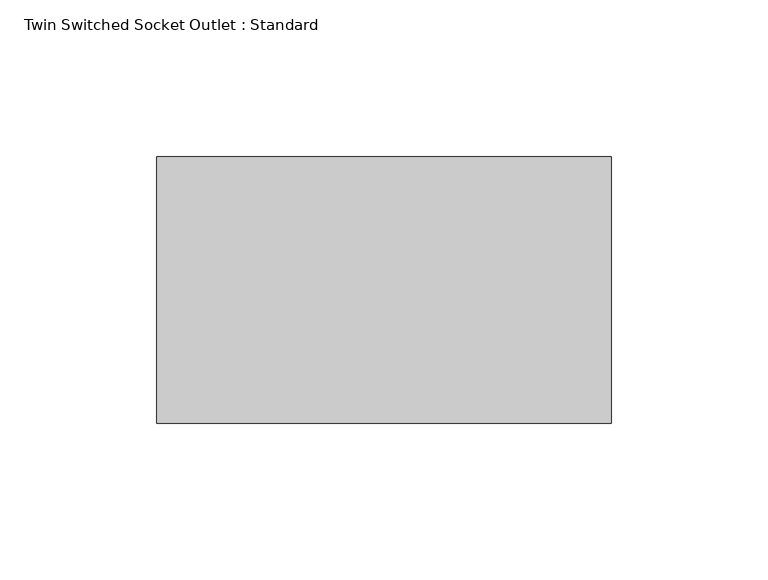
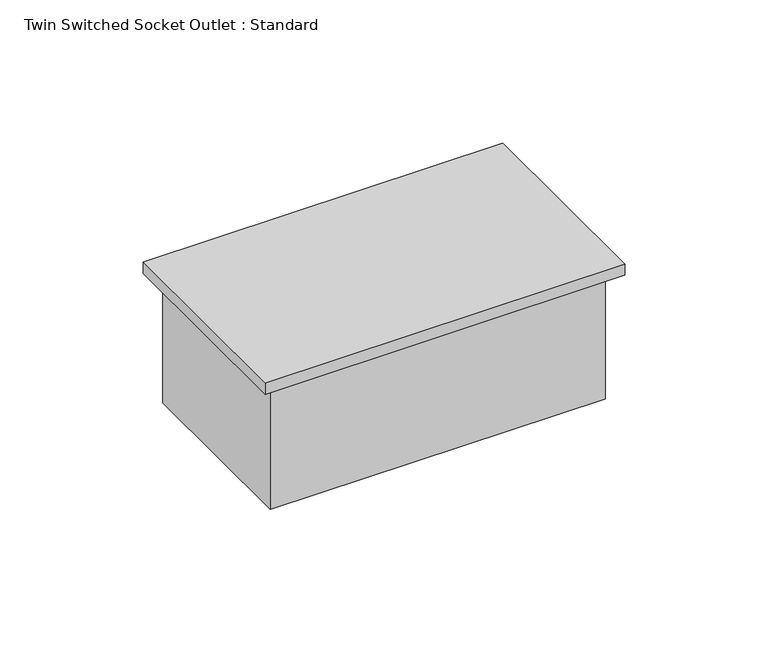
"""IFC4 building model written with IfcOpenShell, lengths in millimetres: proxy geometry, Twin Switched Socket Outlet : Standard."""

from ifc_helpers import new_model, si_unit, frame, origin, origin_with_axes, place, context, project, spatial, polyline, outline, extrude, source, transform, mapped, element, save


def twin_switched_socket_outlet_standard_0deee84c(model_context):
    return source(origin(), model_context, "Body", "SweptSolid", [
        extrude(outline(polyline([(67.5, 37.5), (67.5, -37.5), (-67.5, -37.5), (-67.5, 37.5), (67.5, 37.5)])), frame((0.0, 0.0, -53.975), z_axis=(0.0, 0.0, 1.0), x_axis=(1.0, 0.0, 0.0)), (0.0, 0.0, 1.0), 53.975),
        extrude(outline(polyline([(72.5, 42.5), (72.5, -42.5), (-72.5, -42.5), (-72.5, 42.5), (72.5, 42.5)])), origin_with_axes(), (0.0, 0.0, 1.0), 4.7625),
    ])


if __name__ == "__main__":
    model = new_model("IFC4")
    model_context = context("Model", 3, world=origin())
    ifc_project = project(units=[si_unit("LENGTHUNIT", "METRE", prefix="MILLI")], contexts=[model_context])
    site = spatial("IfcSite", under=ifc_project)
    building = spatial("IfcBuilding", under=site)
    placement = place(None, origin())
    twin_switched_socket_outlet_standard_shape = twin_switched_socket_outlet_standard_0deee84c(model_context)
    element("IfcBuildingElementProxy", 1, Name="Twin Switched Socket Outlet : Standard", ObjectType="Twin Switched Socket Outlet : Standard", at=placement, inside=building, context=model_context, shape_type="MappedRepresentation", body=[
        mapped(twin_switched_socket_outlet_standard_shape, transform((0.0, 0.0, 0.0), x_axis=(1.0, 0.0, 0.0), y_axis=(0.0, 1.0, 0.0), z_axis=(0.0, 0.0, 1.0))),
    ])
    save(model, "model.ifc")

# Revit data of these elements
# Type "Twin Switched Socket Outlet : Standard"
#   Label = "2"
#   Switch Voltage = 230 V
#   Load = 180 VA
#   Default Elevation = 1200 mm
#   Load Classification = Socket
#   Assembly Code = ""
